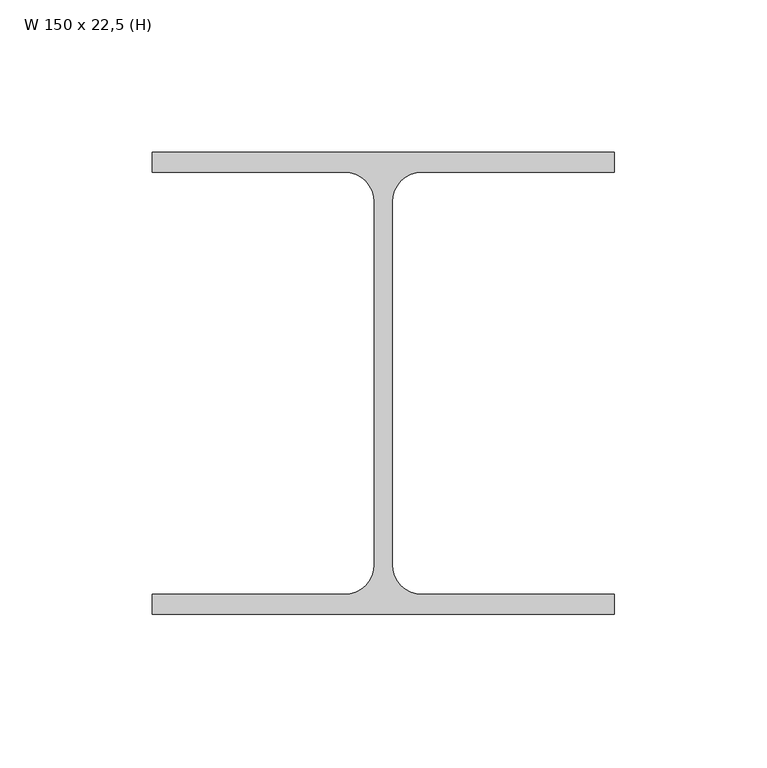
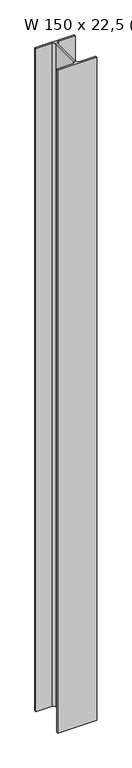
"""IFC4 building model written with IfcOpenShell, lengths in millimetres: column geometry, Pilar de Aço - H : W 150 x 22,5 (H)."""

from ifc_helpers import new_model, si_unit, point, frame_2d, origin, origin_with_axes, place, context, project, spatial, polyline, circle_curve, trimmed, segment, composite_curve, outline, extrude, source, transform, mapped, element, save


def w_150_x_22_5_h_f3c0cc8a(model_context):
    return source(origin(), model_context, "Body", "SweptSolid", [
        extrude(outline(composite_curve([segment(polyline([(76.0, 76.0), (76.0, 69.4), (12.8, 69.4)]), True, "CONTINUOUS"), segment(trimmed(circle_curve(frame_2d((12.8, 59.5)), 9.9), [point((12.8, 69.4))], [point((2.9, 59.5))], True, "CARTESIAN"), True, "CONTINUOUS"), segment(polyline([(2.9, 59.5), (2.9, -59.5)]), True, "CONTINUOUS"), segment(trimmed(circle_curve(frame_2d((12.8, -59.5)), 9.9), [point((2.9, -59.5))], [point((12.8, -69.4))], True, "CARTESIAN"), True, "CONTINUOUS"), segment(polyline([(12.8, -69.4), (76.0, -69.4), (76.0, -76.0), (-76.0, -76.0), (-76.0, -69.4), (-12.8, -69.4)]), True, "CONTINUOUS"), segment(trimmed(circle_curve(frame_2d((-12.8, -59.5)), 9.9), [point((-12.8, -69.4))], [point((-2.9, -59.5))], True, "CARTESIAN"), True, "CONTINUOUS"), segment(polyline([(-2.9, -59.5), (-2.9, 59.5)]), True, "CONTINUOUS"), segment(trimmed(circle_curve(frame_2d((-12.8, 59.5)), 9.9), [point((-2.9, 59.5))], [point((-12.8, 69.4))], True, "CARTESIAN"), True, "CONTINUOUS"), segment(polyline([(-12.8, 69.4), (-76.0, 69.4), (-76.0, 76.0), (76.0, 76.0)]), True, "CONTINUOUS")], self_intersect=False)), origin_with_axes(), (0.0, 0.0, 1.0), 2720.0),
    ])


if __name__ == "__main__":
    model = new_model("IFC4")
    model_context = context("Model", 3, world=origin())
    ifc_project = project(units=[si_unit("LENGTHUNIT", "METRE", prefix="MILLI")], contexts=[model_context])
    site = spatial("IfcSite", under=ifc_project)
    building = spatial("IfcBuilding", under=site)
    placement = place(None, origin())
    w_150_x_22_5_h_shape = w_150_x_22_5_h_f3c0cc8a(model_context)
    element("IfcColumn", 1, ObjectType="Pilar de Aço - H : W 150 x 22,5 (H)", at=placement, inside=building, context=model_context, shape_type="MappedRepresentation", body=[
        mapped(w_150_x_22_5_h_shape, transform((0.0, 0.0, 0.0), x_axis=(1.0, 0.0, 0.0), y_axis=(0.0, 1.0, 0.0), z_axis=(0.0, 0.0, 1.0))),
    ])
    save(model, "model.ifc")

# Revit data of these elements
# Type "Pilar de Aço - H : W 150 x 22,5 (H)"
#   SINAPI = ""
#   Área da seção = 29 m²
#   tw = 0.58 cm
#   tf = 0.66 cm
#   h = 13.88 cm
#   d' = 11.90 cm
#   d = 15.20 cm
#   bf = 15.20 cm
#   R = 0.99 cm
#   Massa Linear kg/m = 22.5
#   Aço = Metal - Aço 345MPa
#   Assembly Code = ""
# Materials
#   "Metal - Aço 345MPa": class "Metal", colour RGB 189 187 185, transparency 0, Cost = 0
